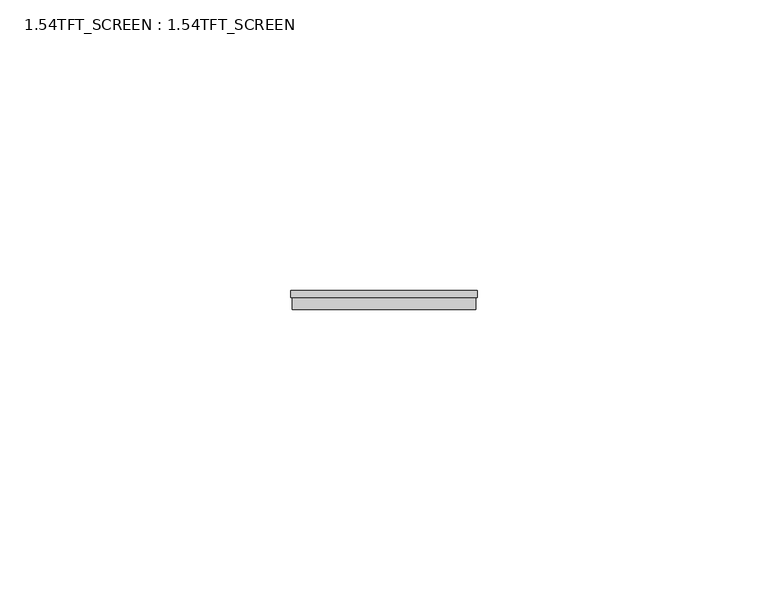
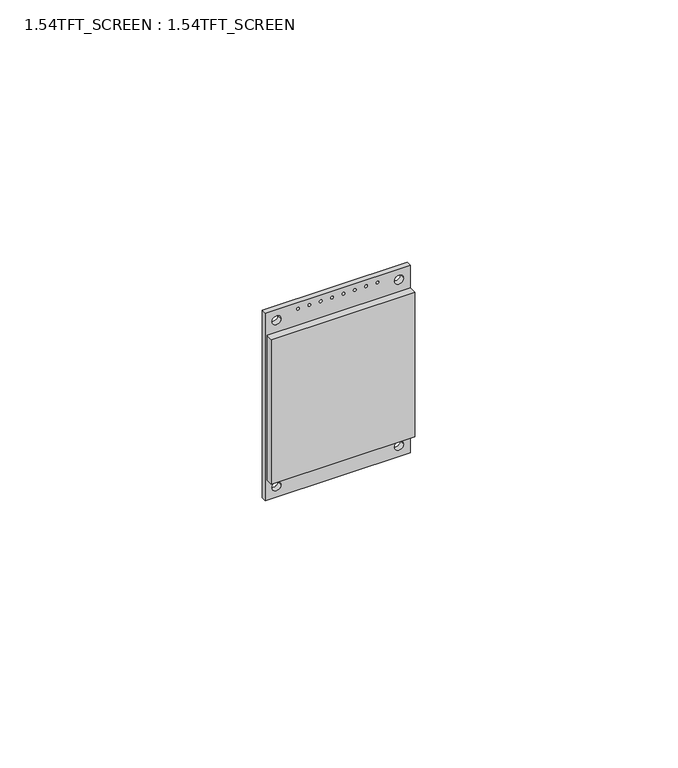
"""IFC4 building model written with IfcOpenShell, lengths in millimetres: furniture geometry, 1.54TFT_SCREEN : 1.54TFT_SCREEN."""

from ifc_helpers import new_model, si_unit, point, frame, frame_2d, origin, place, context, project, spatial, polyline, circle_curve, trimmed, segment, composite_curve, outline, extrude, source, transform, mapped, element, save


def furniture_1_54tft_screen_1_54tft_screen_d9e98271(model_context):
    return source(origin(), model_context, "Body", "SweptSolid", [
        extrude(outline(polyline([(43.7, 16.0), (43.7, -16.0), (0.0, -16.0), (0.0, 16.0), (43.7, 16.0)]), holes=[composite_curve([segment(trimmed(circle_curve(frame_2d((2.5, 13.5)), 1.0), [point((2.5, 14.5))], [point((2.5, 12.5))], True, "CARTESIAN"), True, "CONTINUOUS"), segment(trimmed(circle_curve(frame_2d((2.5, 13.5)), 1.0), [point((2.5, 12.5))], [point((2.5, 14.5))], True, "CARTESIAN"), True, "CONTINUOUS")], self_intersect=False), composite_curve([segment(trimmed(circle_curve(frame_2d((41.2, 13.5)), 1.0), [point((41.2, 14.5))], [point((41.2, 12.5))], True, "CARTESIAN"), True, "CONTINUOUS"), segment(trimmed(circle_curve(frame_2d((41.2, 13.5)), 1.0), [point((41.2, 12.5))], [point((41.2, 14.5))], True, "CARTESIAN"), True, "CONTINUOUS")], self_intersect=False), composite_curve([segment(trimmed(circle_curve(frame_2d((42.2, -1.25)), 0.3), [point((42.2, -0.95))], [point((42.2, -1.55))], True, "CARTESIAN"), True, "CONTINUOUS"), segment(trimmed(circle_curve(frame_2d((42.2, -1.25)), 0.3), [point((42.2, -1.55))], [point((42.2, -0.95))], True, "CARTESIAN"), True, "CONTINUOUS")], self_intersect=False), composite_curve([segment(trimmed(circle_curve(frame_2d((42.2, 1.25)), 0.3), [point((42.2, 1.55))], [point((42.2, 0.95))], True, "CARTESIAN"), True, "CONTINUOUS"), segment(trimmed(circle_curve(frame_2d((42.2, 1.25)), 0.3), [point((42.2, 0.95))], [point((42.2, 1.55))], True, "CARTESIAN"), True, "CONTINUOUS")], self_intersect=False), composite_curve([segment(trimmed(circle_curve(frame_2d((42.2, 3.75)), 0.3), [point((42.2, 4.05))], [point((42.2, 3.45))], True, "CARTESIAN"), True, "CONTINUOUS"), segment(trimmed(circle_curve(frame_2d((42.2, 3.75)), 0.3), [point((42.2, 3.45))], [point((42.2, 4.05))], True, "CARTESIAN"), True, "CONTINUOUS")], self_intersect=False), composite_curve([segment(trimmed(circle_curve(frame_2d((42.2, 6.25)), 0.3), [point((42.2, 6.55))], [point((42.2, 5.95))], True, "CARTESIAN"), True, "CONTINUOUS"), segment(trimmed(circle_curve(frame_2d((42.2, 6.25)), 0.3), [point((42.2, 5.95))], [point((42.2, 6.55))], True, "CARTESIAN"), True, "CONTINUOUS")], self_intersect=False), composite_curve([segment(trimmed(circle_curve(frame_2d((42.2, 8.75)), 0.3), [point((42.2, 9.05))], [point((42.2, 8.45))], True, "CARTESIAN"), True, "CONTINUOUS"), segment(trimmed(circle_curve(frame_2d((42.2, 8.75)), 0.3), [point((42.2, 8.45))], [point((42.2, 9.05))], True, "CARTESIAN"), True, "CONTINUOUS")], self_intersect=False), composite_curve([segment(trimmed(circle_curve(frame_2d((42.2, -3.75)), 0.3), [point((42.2, -3.45))], [point((42.2, -4.05))], True, "CARTESIAN"), True, "CONTINUOUS"), segment(trimmed(circle_curve(frame_2d((42.2, -3.75)), 0.3), [point((42.2, -4.05))], [point((42.2, -3.45))], True, "CARTESIAN"), True, "CONTINUOUS")], self_intersect=False), composite_curve([segment(trimmed(circle_curve(frame_2d((42.2, -6.25)), 0.3), [point((42.2, -5.95))], [point((42.2, -6.55))], True, "CARTESIAN"), True, "CONTINUOUS"), segment(trimmed(circle_curve(frame_2d((42.2, -6.25)), 0.3), [point((42.2, -6.55))], [point((42.2, -5.95))], True, "CARTESIAN"), True, "CONTINUOUS")], self_intersect=False), composite_curve([segment(trimmed(circle_curve(frame_2d((42.2, -8.75)), 0.3), [point((42.2, -8.45))], [point((42.2, -9.05))], True, "CARTESIAN"), True, "CONTINUOUS"), segment(trimmed(circle_curve(frame_2d((42.2, -8.75)), 0.3), [point((42.2, -9.05))], [point((42.2, -8.45))], True, "CARTESIAN"), True, "CONTINUOUS")], self_intersect=False), composite_curve([segment(trimmed(circle_curve(frame_2d((41.2, -13.5)), 1.0), [point((41.2, -14.5))], [point((41.2, -12.5))], True, "CARTESIAN"), True, "CONTINUOUS"), segment(trimmed(circle_curve(frame_2d((41.2, -13.5)), 1.0), [point((41.2, -12.5))], [point((41.2, -14.5))], True, "CARTESIAN"), True, "CONTINUOUS")], self_intersect=False), composite_curve([segment(trimmed(circle_curve(frame_2d((2.5, -13.5)), 1.0), [point((2.5, -14.5))], [point((2.5, -12.5))], True, "CARTESIAN"), True, "CONTINUOUS"), segment(trimmed(circle_curve(frame_2d((2.5, -13.5)), 1.0), [point((2.5, -12.5))], [point((2.5, -14.5))], True, "CARTESIAN"), True, "CONTINUOUS")], self_intersect=False)]), frame((0.0, -1.2, 0.0), z_axis=(0.0, 1.0, 0.0), x_axis=(0.0, 0.0, 1.0)), (0.0, 0.0, 1.0), 1.2),
        extrude(outline(polyline([(15.76, -1.3), (15.76, -3.2), (-15.76, -3.2), (-15.76, -1.3), (15.76, -1.3)])), frame((0.0, 0.0, 5.0), z_axis=(0.0, 0.0, 1.0), x_axis=(1.0, 0.0, 0.0)), (0.0, 0.0, 1.0), 33.7),
        extrude(outline(polyline([(13.86, -2.3592442), (13.86, -3.2), (-13.86, -3.2), (-13.86, -2.3592442), (13.86, -2.3592442)])), frame((0.0, 0.0, 9.5994076), z_axis=(0.0, 0.0, 1.0), x_axis=(1.0, 0.0, 0.0)), (0.0, 0.0, 1.0), 27.7),
    ])


if __name__ == "__main__":
    model = new_model("IFC4")
    model_context = context("Model", 3, world=origin())
    ifc_project = project(units=[si_unit("LENGTHUNIT", "METRE", prefix="MILLI")], contexts=[model_context])
    site = spatial("IfcSite", under=ifc_project)
    building = spatial("IfcBuilding", under=site)
    placement = place(None, origin())
    furniture_1_54tft_screen_1_54tft_screen_shape = furniture_1_54tft_screen_1_54tft_screen_d9e98271(model_context)
    element("IfcFurniture", 1, ObjectType="1.54TFT_SCREEN : 1.54TFT_SCREEN", at=placement, inside=building, context=model_context, shape_type="MappedRepresentation", body=[
        mapped(furniture_1_54tft_screen_1_54tft_screen_shape, transform((0.0, 0.0, 0.0), x_axis=(1.0, 0.0, 0.0), y_axis=(0.0, 1.0, 0.0), z_axis=(0.0, 0.0, 1.0))),
    ])
    save(model, "model.ifc")

# Revit data of these elements
# Type "1.54TFT_SCREEN : 1.54TFT_SCREEN"
#   Default Elevation = 0
# Element 1 (IfcFurniture, "1.54TFT_SCREEN : 1.54TFT_SCREEN")
#   Materials on its faces: ".VIDRO"
# Materials
#   ".VIDRO": class "Vidro", colour RGB 165 190 164, transparency 0.4, Cost = 0
